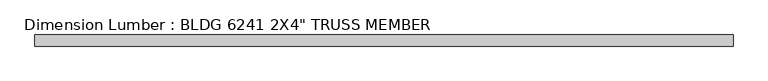
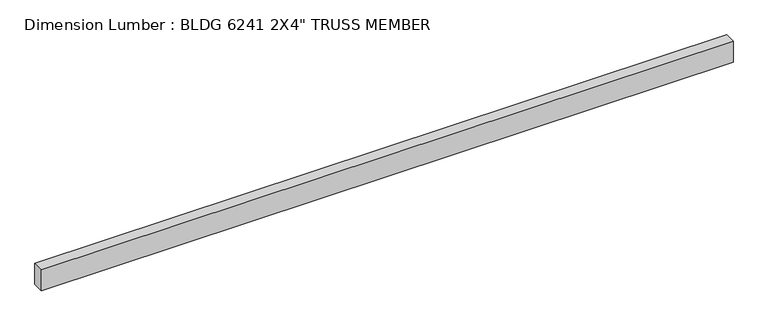
"""IFC4 building model written with IfcOpenShell, lengths in millimetres: beam geometry."""

from ifc_helpers import new_model, si_unit, frame, origin, place, context, project, spatial, polyline, outline, extrude, source, transform, mapped, element, save


def beam_189f326c(model_context):
    return source(origin(), model_context, "Body", "SweptSolid", [
        extrude(outline(polyline([(1574.4380265, 25.4), (1574.4380265, -25.4), (-1601.4606477, -25.4), (-1601.4606477, 25.4), (1574.4380265, 25.4)])), frame((0.0, 0.0, -50.8), z_axis=(0.0, 0.0, 1.0), x_axis=(1.0, 0.0, 0.0)), (0.0, 0.0, 1.0), 101.6),
    ])


if __name__ == "__main__":
    model = new_model("IFC4")
    model_context = context("Model", 3, world=origin())
    ifc_project = project(units=[si_unit("LENGTHUNIT", "METRE", prefix="MILLI")], contexts=[model_context])
    site = spatial("IfcSite", under=ifc_project)
    building = spatial("IfcBuilding", under=site)
    placement = place(None, origin())
    beam_shape = beam_189f326c(model_context)
    element("IfcBeam", 1, ObjectType="Dimension Lumber : BLDG 6241 2X4\" TRUSS MEMBER", at=placement, inside=building, context=model_context, shape_type="MappedRepresentation", body=[
        mapped(beam_shape, transform((0.0, 0.0, 0.0), x_axis=(1.0, 0.0, 0.0), y_axis=(0.0, 1.0, 0.0), z_axis=(0.0, 0.0, 1.0))),
    ])
    save(model, "model.ifc")

# Revit data of these elements
# Type "Dimension Lumber : BLDG 6241 2X4\" TRUSS MEMBER"
#   Assembly Code = "B10"
#   A = 0.273472 SF
#   Length [instance default] = 5' - 0"
#   b = 0' - 2"
#   d = 0' - 4"
#   Structural Material [instance default] = Softwood, Lumber
# Element 1 (IfcBeam, "Dimension Lumber : BLDG 6241 2X4\" TRUSS MEMBER")
#   Materials on its faces: "Softwood, Lumber"
# Materials
#   "Softwood, Lumber": class "Wood", colour RGB 223 192 134, transparency 0, Description = "Pinus Echinata", Cost = 0
